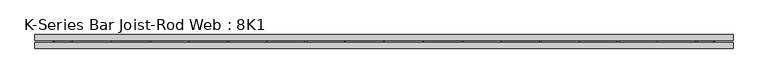
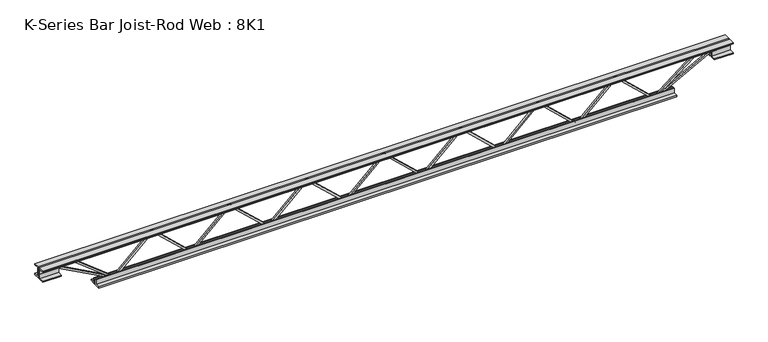
"""IFC4 building model written with IfcOpenShell, lengths in millimetres: beam geometry, K-Series Bar Joist-Rod Web : 8K1."""

from ifc_helpers import new_model, si_unit, frame, origin, place, context, project, spatial, polyline, outline, extrude, source, transform, mapped, element, save


def k_series_bar_joist_rod_web_8k1_67cc681e(model_context):
    return source(origin(), model_context, "Body", "SweptSolid", [
        extrude(outline(polyline([(-90.4875, 629.4128318), (-100.0125, 629.4128318), (-100.0125, 634.4694324), (90.4875, 837.9237097), (90.4875, 840.5105084), (-100.0125, 1043.9647856), (-100.0125, 1049.0213863), (-90.4875, 1049.0213863), (-90.4875, 1047.7279869), (100.0125, 844.2737097), (100.0125, 834.1605084), (-90.4875, 630.7062311), (-90.4875, 629.4128318)])), frame((0.0, -4.7625, 0.0), z_axis=(0.0, 1.0, 0.0), x_axis=(0.0, 0.0, 1.0)), (0.0, 0.0, 1.0), 9.525),
        extrude(outline(polyline([(-90.4875, 209.8042773), (-100.0125, 209.8042773), (-100.0125, 214.8608779), (90.4875, 418.3151552), (90.4875, 420.9019538), (-100.0125, 624.3562311), (-100.0125, 629.4128318), (-90.4875, 629.4128318), (-90.4875, 628.1194324), (100.0125, 424.6651552), (100.0125, 414.5519538), (-90.4875, 211.0976766), (-90.4875, 209.8042773)])), frame((0.0, -4.7625, 0.0), z_axis=(0.0, 1.0, 0.0), x_axis=(0.0, 0.0, 1.0)), (0.0, 0.0, 1.0), 9.525),
        extrude(outline(polyline([(-90.4875, -209.8042773), (-100.0125, -209.8042773), (-100.0125, -204.7476766), (90.4875, -1.2933993), (90.4875, 1.2933993), (-100.0125, 204.7476766), (-100.0125, 209.8042773), (-90.4875, 209.8042773), (-90.4875, 208.5108779), (100.0125, 5.0566007), (100.0125, -5.0566007), (-90.4875, -208.5108779), (-90.4875, -209.8042773)])), frame((0.0, -4.7625, 0.0), z_axis=(0.0, 1.0, 0.0), x_axis=(0.0, 0.0, 1.0)), (0.0, 0.0, 1.0), 9.525),
        extrude(outline(polyline([(-90.4875, -629.4128318), (-100.0125, -629.4128318), (-100.0125, -624.3562311), (90.4875, -420.9019538), (90.4875, -418.3151552), (-100.0125, -214.8608779), (-100.0125, -209.8042773), (-90.4875, -209.8042773), (-90.4875, -211.0976766), (100.0125, -414.5519538), (100.0125, -424.6651552), (-90.4875, -628.1194324), (-90.4875, -629.4128318)])), frame((0.0, -4.7625, 0.0), z_axis=(0.0, 1.0, 0.0), x_axis=(0.0, 0.0, 1.0)), (0.0, 0.0, 1.0), 9.525),
        extrude(outline(polyline([(-90.4875, -1049.0213863), (-100.0125, -1049.0213863), (-100.0125, -1043.9647856), (90.4875, -840.5105084), (90.4875, -837.9237097), (-100.0125, -634.4694324), (-100.0125, -629.4128318), (-90.4875, -629.4128318), (-90.4875, -630.7062311), (100.0125, -834.1605084), (100.0125, -844.2737097), (-90.4875, -1047.7279869), (-90.4875, -1049.0213863)])), frame((0.0, -4.7625, 0.0), z_axis=(0.0, 1.0, 0.0), x_axis=(0.0, 0.0, 1.0)), (0.0, 0.0, 1.0), 9.525),
        extrude(outline(polyline([(-90.4875, 1049.0213863), (-100.0125, 1049.0213863), (-100.0125, 1054.0779869), (90.4875, 1257.5322642), (90.4875, 1260.1190629), (-100.0125, 1463.5733401), (-100.0125, 1468.6299408), (-90.4875, 1468.6299408), (-90.4875, 1467.3365415), (100.0125, 1263.8822642), (100.0125, 1253.7690629), (-90.4875, 1050.3147856), (-90.4875, 1049.0213863)])), frame((0.0, -4.7625, 0.0), z_axis=(0.0, 1.0, 0.0), x_axis=(0.0, 0.0, 1.0)), (0.0, 0.0, 1.0), 9.525),
        extrude(outline(polyline([(-90.4875, -1468.6299408), (-100.0125, -1468.6299408), (-100.0125, -1463.5733401), (90.4875, -1260.1190629), (90.4875, -1257.5322642), (-100.0125, -1054.0779869), (-100.0125, -1049.0213863), (-90.4875, -1049.0213863), (-90.4875, -1050.3147856), (100.0125, -1253.7690629), (100.0125, -1263.8822642), (-90.4875, -1467.3365415), (-90.4875, -1468.6299408)])), frame((0.0, -4.7625, 0.0), z_axis=(0.0, 1.0, 0.0), x_axis=(0.0, 0.0, 1.0)), (0.0, 0.0, 1.0), 9.525),
        extrude(outline(polyline([(4.7625, 101.6), (36.5125, 101.6), (36.5125, 95.25), (11.1125, 95.25), (11.1125, 69.85), (4.7625, 69.85), (4.7625, 101.6)])), frame((-1875.0299408, 0.0, 0.0), z_axis=(1.0, 0.0, 0.0), x_axis=(0.0, 1.0, 0.0)), (0.0, 0.0, 1.0), 3750.0598816),
        extrude(outline(polyline([(-4.7625, 101.6), (-4.7625, 69.85), (-11.1125, 69.85), (-11.1125, 95.25), (-36.5125, 95.25), (-36.5125, 101.6), (-4.7625, 101.6)])), frame((-1875.0299408, 0.0, 0.0), z_axis=(1.0, 0.0, 0.0), x_axis=(0.0, 1.0, 0.0)), (0.0, 0.0, 1.0), 3750.0598816),
        extrude(outline(polyline([(-4.7625, 38.1), (-36.5125, 38.1), (-36.5125, 44.45), (-11.1125, 44.45), (-11.1125, 69.85), (-4.7625, 69.85), (-4.7625, 38.1)])), frame((-1875.0299408, 0.0, 0.0), z_axis=(1.0, 0.0, 0.0), x_axis=(0.0, 1.0, 0.0)), (0.0, 0.0, 1.0), 101.6),
        extrude(outline(polyline([(36.5125, 38.1), (4.7625, 38.1), (4.7625, 69.85), (11.1125, 69.85), (11.1125, 44.45), (36.5125, 44.45), (36.5125, 38.1)])), frame((-1875.0299408, 0.0, 0.0), z_axis=(1.0, 0.0, 0.0), x_axis=(0.0, 1.0, 0.0)), (0.0, 0.0, 1.0), 101.6),
        extrude(outline(polyline([(4.7625, 38.1), (4.7625, 69.85), (11.1125, 69.85), (11.1125, 44.45), (36.5125, 44.45), (36.5125, 38.1), (4.7625, 38.1)])), frame((1773.4299408, 0.0, 0.0), z_axis=(1.0, 0.0, 0.0), x_axis=(0.0, 1.0, 0.0)), (0.0, 0.0, 1.0), 101.6),
        extrude(outline(polyline([(-4.7625, 38.1), (-36.5125, 38.1), (-36.5125, 44.45), (-11.1125, 44.45), (-11.1125, 69.85), (-4.7625, 69.85), (-4.7625, 38.1)])), frame((1773.4299408, 0.0, 0.0), z_axis=(1.0, 0.0, 0.0), x_axis=(0.0, 1.0, 0.0)), (0.0, 0.0, 1.0), 101.6),
        extrude(outline(polyline([(4.7625, -101.6), (4.7625, -69.85), (11.1125, -69.85), (11.1125, -95.25), (36.5125, -95.25), (36.5125, -101.6), (4.7625, -101.6)])), frame((-1570.2299408, 0.0, 0.0), z_axis=(1.0, 0.0, 0.0), x_axis=(0.0, 1.0, 0.0)), (0.0, 0.0, 1.0), 3140.4598816),
        extrude(outline(polyline([(-4.7625, -101.6), (-36.5125, -101.6), (-36.5125, -95.25), (-11.1125, -95.25), (-11.1125, -69.85), (-4.7625, -69.85), (-4.7625, -101.6)])), frame((-1570.2299408, 0.0, 0.0), z_axis=(1.0, 0.0, 0.0), x_axis=(0.0, 1.0, 0.0)), (0.0, 0.0, 1.0), 3140.4598816),
        extrude(outline(polyline([(0.0, -9.525), (0.0, 0.0), (346.6425392, 0.0), (346.6425392, -9.525), (0.0, -9.525)])), frame((-1775.6982393, 4.7625, 65.662372), z_axis=(0.47628314854007936, 0.0, 0.8792919665371388), x_axis=(0.8792919665371388, 0.0, -0.47628314854007936)), (0.0, 0.0, 1.0), 9.525),
        extrude(outline(polyline([(0.0, -9.525), (0.0, 0.0), (266.9753636, 0.0), (266.9753636, -9.525), (0.0, -9.525)])), frame((-1681.3793915, 4.7625, 66.1073593), z_axis=(0.6184091213150067, 0.0, 0.7858563219026754), x_axis=(0.7858563219026754, 0.0, -0.6184091213150067)), (0.0, 0.0, 1.0), 9.525),
        extrude(outline(polyline([(0.0, -9.525), (0.0, 0.0), (346.6425392, 0.0), (346.6425392, -9.525), (0.0, -9.525)])), frame((1775.6982393, -4.7625, 65.662372), z_axis=(-0.47628314854004167, 0.0, 0.8792919665371591), x_axis=(-0.8792919665371591, 0.0, -0.47628314854004167)), (0.0, 0.0, 1.0), 9.525),
        extrude(outline(polyline([(0.0, -9.525), (0.0, 0.0), (266.9753636, 0.0), (266.9753636, -9.525), (0.0, -9.525)])), frame((1681.3793915, -4.7625, 66.1073593), z_axis=(-0.6184091213149836, 0.0, 0.7858563219026936), x_axis=(-0.7858563219026936, 0.0, -0.6184091213149836)), (0.0, 0.0, 1.0), 9.525),
    ])


if __name__ == "__main__":
    model = new_model("IFC4")
    model_context = context("Model", 3, world=origin())
    ifc_project = project(units=[si_unit("LENGTHUNIT", "METRE", prefix="MILLI")], contexts=[model_context])
    site = spatial("IfcSite", under=ifc_project)
    building = spatial("IfcBuilding", under=site)
    placement = place(None, origin())
    k_series_bar_joist_rod_web_8k1_shape = k_series_bar_joist_rod_web_8k1_67cc681e(model_context)
    element("IfcBeam", 1, ObjectType="K-Series Bar Joist-Rod Web : 8K1", at=placement, inside=building, context=model_context, shape_type="MappedRepresentation", body=[
        mapped(k_series_bar_joist_rod_web_8k1_shape, transform((0.0, 0.0, 0.0), x_axis=(1.0, 0.0, 0.0), y_axis=(0.0, 1.0, 0.0), z_axis=(0.0, 0.0, 1.0))),
    ])
    save(model, "model.ifc")

# Revit data of these elements
# Type "K-Series Bar Joist-Rod Web : 8K1"
#   Assembly Code = "B1010350"
#   Wt = 5.1
#   Web Thickness = 0' - 0 3/8"
#   Start Offset [instance default] = 0' - 0"
#   Start Extension [instance default] = 0' - 0"
#   Seat Length = 0' - 4"
#   Seat Depth = 0' - 2 1/2"
#   PanelArrayLength [instance default] = 21' - 4"
#   Panel [instance default] = 1' - 4"
#   End Offset [instance default] = 0' - 0"
#   End Extension [instance default] = 0' - 0"
#   End Panel = 1' - 4"
#   Cord Leg = 0' - 1 1/4"
#   Chord Thickness = 0' - 0 1/4"
#   Length [instance default] = 24' - 0"
#   Depth = 0' - 8"
#   PanelArrayNum [instance default] = 16
#   Rendering Material = none
# Element 1 (IfcBeam, "K-Series Bar Joist-Rod Web : 8K1")
#   PanelArrayLength = 9' - 7.64015"
#   Panel = 1' - 4.52002"
#   PanelArrayNum = 7
